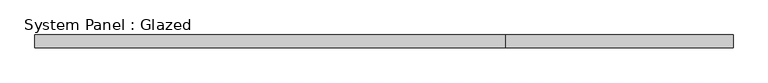
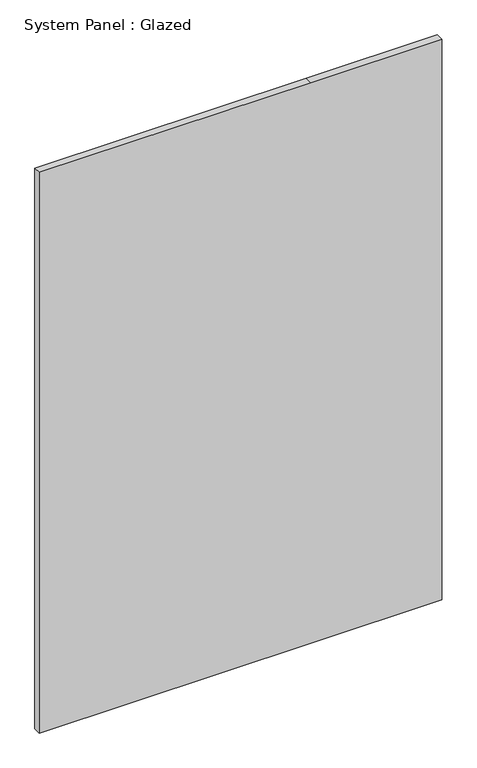
"""IFC4 building model written with IfcOpenShell, lengths in millimetres: plate geometry, System Panel : Glazed."""

from ifc_helpers import new_model, si_unit, frame, origin, place, context, project, spatial, polyline, outline, extrude, source, transform, mapped, element, save


def system_panel_glazed_b2aaa3aa(model_context):
    return source(origin(), model_context, "Body", "SweptSolid", [
        extrude(outline(polyline([(0.0, -692.15), (0.0, 241.3), (0.0, 692.15), (2038.35, 692.15), (2038.35, 241.3), (2038.35, -692.15), (0.0, -692.15)])), frame((0.0, -44.45, 0.0), z_axis=(0.0, 1.0, 0.0), x_axis=(0.0, 0.0, 1.0)), (0.0, 0.0, 1.0), 25.4),
    ])


if __name__ == "__main__":
    model = new_model("IFC4")
    model_context = context("Model", 3, world=origin())
    ifc_project = project(units=[si_unit("LENGTHUNIT", "METRE", prefix="MILLI")], contexts=[model_context])
    site = spatial("IfcSite", under=ifc_project)
    building = spatial("IfcBuilding", under=site)
    placement = place(None, origin())
    system_panel_glazed_shape = system_panel_glazed_b2aaa3aa(model_context)
    element("IfcPlate", 1, ObjectType="System Panel : Glazed", at=placement, inside=building, context=model_context, shape_type="MappedRepresentation", body=[
        mapped(system_panel_glazed_shape, transform((0.0, 0.0, 0.0), x_axis=(1.0, 0.0, 0.0), y_axis=(0.0, 1.0, 0.0), z_axis=(0.0, 0.0, 1.0))),
    ])
    save(model, "model.ifc")

# Revit data of these elements
# Type "System Panel : Glazed"
#   Construction Type Id = "GSP4R"
#   Analytic Construction = "1/8 in Pilkington single glazing"
#   Visual Light Transmittance = 0.9
#   Solar Heat Gain Coefficient = 0.86
#   Heat Transfer Coefficient (U) = 1.18115 BTU/(h·ft²·°F)
#   Define Thermal Properties by = 1
# Element 1 (IfcPlate, "System Panel : Glazed")
#   Materials on its faces: "Glass"
# Materials
#   "Glass": class "Glass", colour RGB 0 0 255, transparency 0.75, Description = "Soda Lime Glass", Cost = 0
